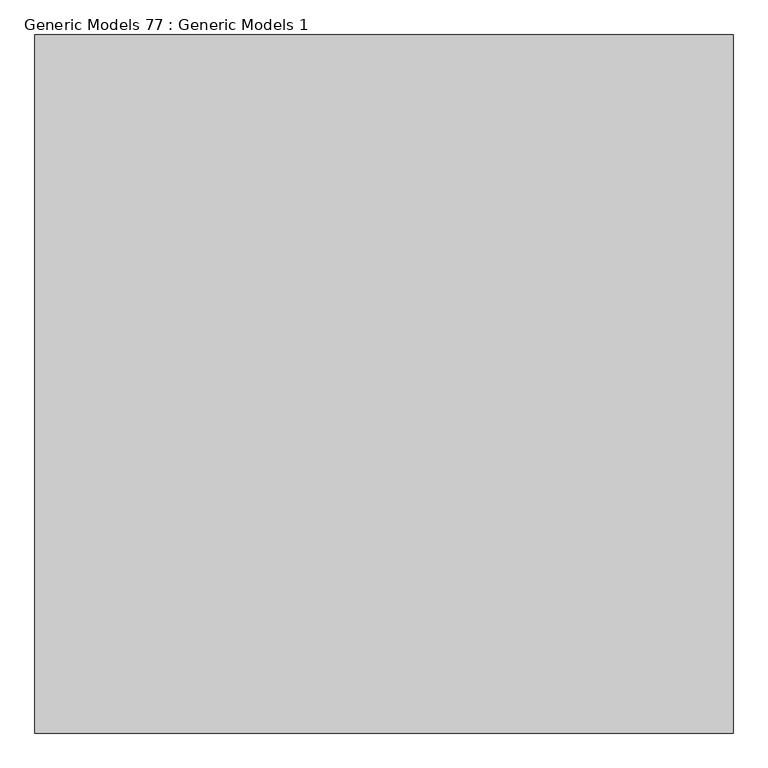
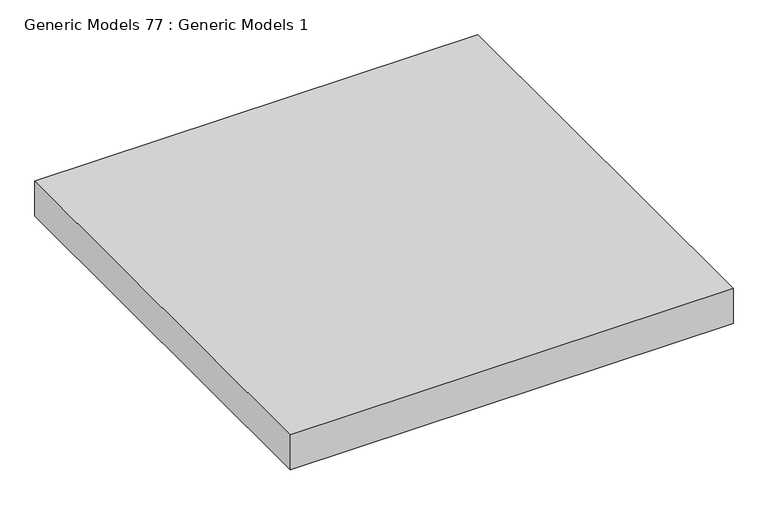
"""IFC4 building model written with IfcOpenShell, lengths in millimetres: proxy geometry, Generic Models 77 : Generic Models 1."""

import ifcopenshell
import ifcopenshell.guid

model = None  # the IFC model being written
_history = None  # IfcOwnerHistory: only IFC2X3 demands one
_inside = {}  # id of a spatial element -> (the spatial element, [elements in it])
_under = {}  # id of a project, library or spatial element -> (it, [spatial elements below it])
_declared = {}  # id of a project -> (the project, [libraries it declares])
_typed = {}  # id of a type object -> (the type object, [elements of that type])
_made_of = {}  # id of a material, layer set ... -> (it, [elements and type objects made of it])


def new_model(schema):
    """Start an empty IFC model of exactly this schema.

    Asked for "IFC4X3", IfcOpenShell would pick the latest addendum, in which some entities
    have other attributes; the version numbers below select the first issue.
    IFC2X3 requires an IfcOwnerHistory on every rooted entity: one is made here for all.
    """
    global model, _history
    if schema == "IFC4X3":
        model = ifcopenshell.file(schema_version=(4, 3, 0, 0))
    else:
        model = ifcopenshell.file(schema=schema)
    _inside.clear()
    _under.clear()
    _declared.clear()
    _typed.clear()
    _made_of.clear()
    _history = None
    if model.schema == "IFC2X3":
        org = make("IfcOrganization", Name="unknown")
        user = make(
            "IfcPersonAndOrganization",
            ThePerson=make("IfcPerson", FamilyName="unknown"),
            TheOrganization=org,
        )
        app = make(
            "IfcApplication",
            ApplicationDeveloper=org,
            Version="unknown",
            ApplicationFullName="unknown",
            ApplicationIdentifier="unknown",
        )
        _history = make(
            "IfcOwnerHistory",
            OwningUser=user,
            OwningApplication=app,
            ChangeAction="ADDED",
            CreationDate=0,
        )
    return model


def make(cls, **values):
    """One entity of the class cls with the attributes given. An attribute that is None is left unset."""
    return model.create_entity(
        cls, **{name: value for name, value in values.items() if value is not None}
    )


def rooted(cls, **values):
    """An entity with a GlobalId (a new one), such as an element, a storey or a relation."""
    return make(cls, GlobalId=ifcopenshell.guid.new(), OwnerHistory=_history, **values)


def si_unit(unit_type, name, prefix=None):
    """IfcSIUnit, for example si_unit("LENGTHUNIT", "METRE", prefix="MILLI")."""
    return make("IfcSIUnit", UnitType=unit_type, Prefix=prefix, Name=name)


def assignment(units):
    """IfcUnitAssignment: the units of a project."""
    return None if units is None else make("IfcUnitAssignment", Units=units)


def point(xyz):
    """IfcCartesianPoint."""
    return None if xyz is None else make("IfcCartesianPoint", Coordinates=xyz)


def direction(xyz):
    """IfcDirection."""
    return None if xyz is None else make("IfcDirection", DirectionRatios=xyz)


def frame(location, z_axis=None, x_axis=None):
    """IfcAxis2Placement3D, a coordinate frame: its origin and axes. An axis left out is left unset."""
    return make(
        "IfcAxis2Placement3D",
        Location=point(location),
        Axis=direction(z_axis),
        RefDirection=direction(x_axis),
    )


def origin():
    """The frame at (0, 0, 0) with its axes left unset."""
    return frame((0.0, 0.0, 0.0))


def place(relative_to, where):
    """IfcLocalPlacement: puts the frame where relative to a parent placement (None: the world)."""
    return make(
        "IfcLocalPlacement", PlacementRelTo=relative_to, RelativePlacement=where
    )


def context(
    kind, dimensions, precision=None, world=None, true_north=None, identifier=None
):
    """IfcGeometricRepresentationContext, for example the 3D "Model" context."""
    return make(
        "IfcGeometricRepresentationContext",
        ContextIdentifier=identifier,
        ContextType=kind,
        CoordinateSpaceDimension=dimensions,
        Precision=precision,
        WorldCoordinateSystem=world,
        TrueNorth=true_north,
    )


def project(units=None, contexts=None):
    """IfcProject with its units and contexts."""
    return rooted(
        "IfcProject",
        Name="project",
        RepresentationContexts=contexts,
        UnitsInContext=assignment(units),
    )


def spatial(cls, under=None, at=None, **own):
    """A site, building, storey or space (cls), placed at a placement, below another one or the project."""
    s = rooted(cls, ObjectPlacement=at, **own)
    if under is not None:
        _under.setdefault(under.id(), (under, []))[1].append(s)
    return s


def polyline(points):
    """IfcPolyline through the points."""
    return make("IfcPolyline", Points=[point(p) for p in points])


def outline(outer, holes=None, kind="AREA"):
    """IfcArbitraryClosedProfileDef: a profile drawn as a closed curve; with holes, ...WithVoids."""
    if holes is None:
        return make("IfcArbitraryClosedProfileDef", ProfileType=kind, OuterCurve=outer)
    return make(
        "IfcArbitraryProfileDefWithVoids",
        ProfileType=kind,
        OuterCurve=outer,
        InnerCurves=holes,
    )


def extrude(swept, where, along, depth):
    """IfcExtrudedAreaSolid: the profile swept, set in the frame where, extruded along a direction by depth."""
    return make(
        "IfcExtrudedAreaSolid",
        SweptArea=swept,
        Position=where,
        ExtrudedDirection=direction(along),
        Depth=depth,
    )


def shape(context_of_items, identifier, shape_type, items):
    """IfcShapeRepresentation: the items that make up one representation, for example the "Body"."""
    return make(
        "IfcShapeRepresentation",
        ContextOfItems=context_of_items,
        RepresentationIdentifier=identifier,
        RepresentationType=shape_type,
        Items=items,
    )


def source(mapping_origin, context_of_items, identifier, shape_type, items):
    """IfcRepresentationMap: a shape defined once, which mapped items show again and again."""
    return make(
        "IfcRepresentationMap",
        MappingOrigin=mapping_origin,
        MappedRepresentation=shape(context_of_items, identifier, shape_type, items),
    )


def transform(
    local_origin,
    x_axis=None,
    y_axis=None,
    z_axis=None,
    scale=None,
    scale2=None,
    scale3=None,
    uniform=True,
):
    """IfcCartesianTransformationOperator3D, or its non-uniform kind. x_axis, y_axis, z_axis: its Axis1, 2, 3."""
    if uniform:
        return make(
            "IfcCartesianTransformationOperator3D",
            Axis1=direction(x_axis),
            Axis2=direction(y_axis),
            LocalOrigin=point(local_origin),
            Scale=scale,
            Axis3=direction(z_axis),
        )
    return make(
        "IfcCartesianTransformationOperator3DnonUniform",
        Axis1=direction(x_axis),
        Axis2=direction(y_axis),
        LocalOrigin=point(local_origin),
        Scale=scale,
        Axis3=direction(z_axis),
        Scale2=scale2,
        Scale3=scale3,
    )


def mapped(mapping_source, mapping_target):
    """IfcMappedItem: shows the shape of a source again, moved by a transform."""
    return make(
        "IfcMappedItem", MappingSource=mapping_source, MappingTarget=mapping_target
    )


def made_of(thing, what):
    """Note that an element or type object is made of a material, layer set ...; save() writes the relation."""
    if what is not None:
        _made_of.setdefault(what.id(), (what, []))[1].append(thing)
    return thing


def element(
    cls,
    number,
    at=None,
    inside=None,
    cuts=None,
    type_object=None,
    material=None,
    context=None,
    identifier="Body",
    shape_type=None,
    held_by="IfcProductDefinitionShape",
    body=None,
    shapes=None,
    **own,
):
    """One element of the class cls, such as IfcWall. Its Tag is "e" and its number.

    at: its placement. inside: the storey or other place that contains it. cuts: it is an
    opening in that element (IfcRelVoidsElement). A single representation is given by context,
    identifier, shape_type and body (its items); several are given by shapes. held_by: the class
    of the entity that holds the representations. save() writes the other relations.
    """
    e = rooted(cls, Tag="e%d" % number, ObjectPlacement=at, **own)
    if body is not None:
        shapes = [shape(context, identifier, shape_type, body)]
    if shapes is not None:
        e.Representation = make(held_by, Representations=shapes)
    if inside is not None:
        _inside.setdefault(inside.id(), (inside, []))[1].append(e)
    if cuts is not None:
        rooted(
            "IfcRelVoidsElement", RelatingBuildingElement=cuts, RelatedOpeningElement=e
        )
    if type_object is not None:
        _typed.setdefault(type_object.id(), (type_object, []))[1].append(e)
    return made_of(e, material)


def aggregate(whole, parts):
    """IfcRelAggregates: a whole, such as a stair, and the parts it consists of."""
    return rooted("IfcRelAggregates", RelatingObject=whole, RelatedObjects=parts)


def save(model, path):
    """Write the relations noted so far, then the file.

    IfcRelAggregates (storeys below a building ...), IfcRelContainedInSpatialStructure (elements
    in a storey), IfcRelDefinesByType, IfcRelAssociatesMaterial and IfcRelDeclares: one each for
    every whole, place, type object, material and project.
    """
    for whole, parts in _under.values():
        aggregate(whole, parts)
    for where, things in _inside.values():
        rooted(
            "IfcRelContainedInSpatialStructure",
            RelatedElements=things,
            RelatingStructure=where,
        )
    for kind, things in _typed.values():
        rooted("IfcRelDefinesByType", RelatedObjects=things, RelatingType=kind)
    for what, things in _made_of.values():
        rooted("IfcRelAssociatesMaterial", RelatedObjects=things, RelatingMaterial=what)
    for by, libraries in _declared.values():
        rooted("IfcRelDeclares", RelatingContext=by, RelatedDefinitions=libraries)
    model.write(path)


def generic_models_77_generic_models_1_8544dbac(model_context):
    return source(origin(), model_context, "Body", "SweptSolid", [
        extrude(outline(polyline([(49128.3625, 0.0), (47909.1625, 0.0), (47909.1625, 1219.2), (49128.3625, 1219.2), (49128.3625, 0.0)])), frame((0.0, 0.0, 2485.300412), z_axis=(0.0, 0.0, 1.0), x_axis=(1.0, 0.0, 0.0)), (0.0, 0.0, 1.0), 101.6),
    ])


if __name__ == "__main__":
    model = new_model("IFC4")
    model_context = context("Model", 3, world=origin())
    ifc_project = project(units=[si_unit("LENGTHUNIT", "METRE", prefix="MILLI")], contexts=[model_context])
    site = spatial("IfcSite", under=ifc_project)
    building = spatial("IfcBuilding", under=site)
    placement = place(None, origin())
    generic_models_77_generic_models_1_shape = generic_models_77_generic_models_1_8544dbac(model_context)
    element("IfcBuildingElementProxy", 1, Name="Generic Models 77 : Generic Models 1", ObjectType="Generic Models 77 : Generic Models 1", at=placement, inside=building, context=model_context, shape_type="MappedRepresentation", body=[
        mapped(generic_models_77_generic_models_1_shape, transform((0.0, 0.0, 0.0), x_axis=(1.0, 0.0, 0.0), y_axis=(0.0, 1.0, 0.0), z_axis=(0.0, 0.0, 1.0))),
    ])
    save(model, "model.ifc")

# Revit data of these elements
# Element 1 (IfcBuildingElementProxy, "Generic Models 77 : Generic Models 1")
#   Materials on its faces: "UNDERSIDE OF STRUCTURE"
# Materials
#   "UNDERSIDE OF STRUCTURE": class "Concrete", colour RGB 115 116 108, transparency 0, Description = "Lightweight concrete", Cost = 0
